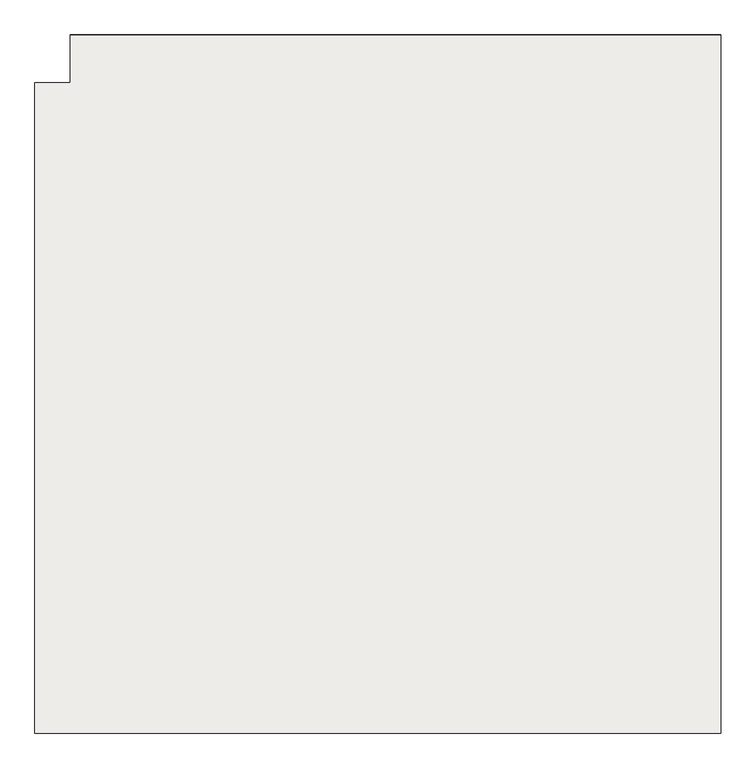
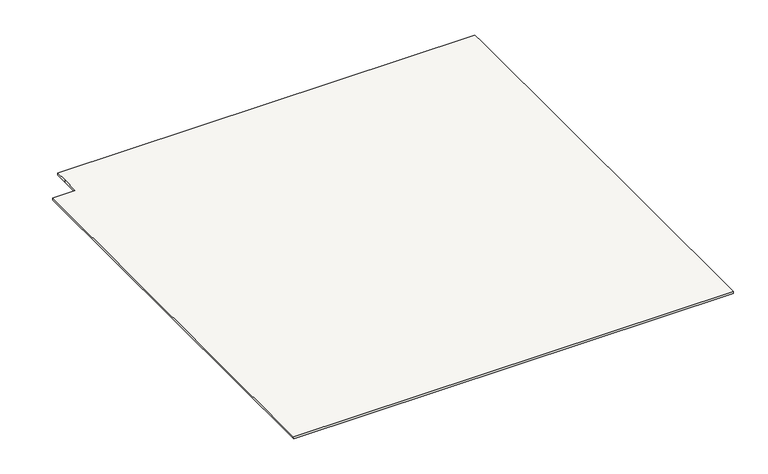
"""IFC4 building model written with IfcOpenShell, lengths in millimetres: slab geometry."""

import ifcopenshell
import ifcopenshell.guid

model = None  # the IFC model being written
_history = None  # IfcOwnerHistory: only IFC2X3 demands one
_inside = {}  # id of a spatial element -> (the spatial element, [elements in it])
_under = {}  # id of a project, library or spatial element -> (it, [spatial elements below it])
_declared = {}  # id of a project -> (the project, [libraries it declares])
_typed = {}  # id of a type object -> (the type object, [elements of that type])
_made_of = {}  # id of a material, layer set ... -> (it, [elements and type objects made of it])


def new_model(schema):
    """Start an empty IFC model of exactly this schema.

    Asked for "IFC4X3", IfcOpenShell would pick the latest addendum, in which some entities
    have other attributes; the version numbers below select the first issue.
    IFC2X3 requires an IfcOwnerHistory on every rooted entity: one is made here for all.
    """
    global model, _history
    if schema == "IFC4X3":
        model = ifcopenshell.file(schema_version=(4, 3, 0, 0))
    else:
        model = ifcopenshell.file(schema=schema)
    _inside.clear()
    _under.clear()
    _declared.clear()
    _typed.clear()
    _made_of.clear()
    _history = None
    if model.schema == "IFC2X3":
        org = make("IfcOrganization", Name="unknown")
        user = make(
            "IfcPersonAndOrganization",
            ThePerson=make("IfcPerson", FamilyName="unknown"),
            TheOrganization=org,
        )
        app = make(
            "IfcApplication",
            ApplicationDeveloper=org,
            Version="unknown",
            ApplicationFullName="unknown",
            ApplicationIdentifier="unknown",
        )
        _history = make(
            "IfcOwnerHistory",
            OwningUser=user,
            OwningApplication=app,
            ChangeAction="ADDED",
            CreationDate=0,
        )
    return model


def make(cls, **values):
    """One entity of the class cls with the attributes given. An attribute that is None is left unset."""
    return model.create_entity(
        cls, **{name: value for name, value in values.items() if value is not None}
    )


def rooted(cls, **values):
    """An entity with a GlobalId (a new one), such as an element, a storey or a relation."""
    return make(cls, GlobalId=ifcopenshell.guid.new(), OwnerHistory=_history, **values)


def si_unit(unit_type, name, prefix=None):
    """IfcSIUnit, for example si_unit("LENGTHUNIT", "METRE", prefix="MILLI")."""
    return make("IfcSIUnit", UnitType=unit_type, Prefix=prefix, Name=name)


def assignment(units):
    """IfcUnitAssignment: the units of a project."""
    return None if units is None else make("IfcUnitAssignment", Units=units)


def point(xyz):
    """IfcCartesianPoint."""
    return None if xyz is None else make("IfcCartesianPoint", Coordinates=xyz)


def direction(xyz):
    """IfcDirection."""
    return None if xyz is None else make("IfcDirection", DirectionRatios=xyz)


def frame(location, z_axis=None, x_axis=None):
    """IfcAxis2Placement3D, a coordinate frame: its origin and axes. An axis left out is left unset."""
    return make(
        "IfcAxis2Placement3D",
        Location=point(location),
        Axis=direction(z_axis),
        RefDirection=direction(x_axis),
    )


def origin():
    """The frame at (0, 0, 0) with its axes left unset."""
    return frame((0.0, 0.0, 0.0))


def place(relative_to, where):
    """IfcLocalPlacement: puts the frame where relative to a parent placement (None: the world)."""
    return make(
        "IfcLocalPlacement", PlacementRelTo=relative_to, RelativePlacement=where
    )


def context(
    kind, dimensions, precision=None, world=None, true_north=None, identifier=None
):
    """IfcGeometricRepresentationContext, for example the 3D "Model" context."""
    return make(
        "IfcGeometricRepresentationContext",
        ContextIdentifier=identifier,
        ContextType=kind,
        CoordinateSpaceDimension=dimensions,
        Precision=precision,
        WorldCoordinateSystem=world,
        TrueNorth=true_north,
    )


def project(units=None, contexts=None):
    """IfcProject with its units and contexts."""
    return rooted(
        "IfcProject",
        Name="project",
        RepresentationContexts=contexts,
        UnitsInContext=assignment(units),
    )


def spatial(cls, under=None, at=None, **own):
    """A site, building, storey or space (cls), placed at a placement, below another one or the project."""
    s = rooted(cls, ObjectPlacement=at, **own)
    if under is not None:
        _under.setdefault(under.id(), (under, []))[1].append(s)
    return s


def faces_of(points, faces, orient=None, outer=None):
    """IfcFace entities. A face is a list of loops; a loop is a list of indices into points, from 0.

    orient and outer hold one flag for each loop. By default every Orientation is true, the
    first loop of a face is its IfcFaceOuterBound and the others are IfcFaceBound.
    """
    made = []
    for i, loops in enumerate(faces):
        bounds = []
        for j, loop in enumerate(loops):
            is_outer = j == 0 if outer is None else outer[i][j]
            bounds.append(
                make(
                    "IfcFaceOuterBound" if is_outer else "IfcFaceBound",
                    Bound=make("IfcPolyLoop", Polygon=[points[k] for k in loop]),
                    Orientation=True if orient is None else orient[i][j],
                )
            )
        made.append(make("IfcFace", Bounds=bounds))
    return made


def faceted_brep(points, faces, orient=None, outer=None, voids=None):
    """IfcFacetedBrep: a solid bounded by flat faces; with voids (closed shells), ...WithVoids."""
    shared = [point(p) for p in points]
    hull = make("IfcClosedShell", CfsFaces=faces_of(shared, faces, orient, outer))
    if voids is None:
        return make("IfcFacetedBrep", Outer=hull)
    return make(
        "IfcFacetedBrepWithVoids",
        Outer=hull,
        Voids=[
            make(cls, CfsFaces=faces_of(shared, fs, o, b)) for cls, fs, o, b in voids
        ],
    )


def shape(context_of_items, identifier, shape_type, items):
    """IfcShapeRepresentation: the items that make up one representation, for example the "Body"."""
    return make(
        "IfcShapeRepresentation",
        ContextOfItems=context_of_items,
        RepresentationIdentifier=identifier,
        RepresentationType=shape_type,
        Items=items,
    )


def source(mapping_origin, context_of_items, identifier, shape_type, items):
    """IfcRepresentationMap: a shape defined once, which mapped items show again and again."""
    return make(
        "IfcRepresentationMap",
        MappingOrigin=mapping_origin,
        MappedRepresentation=shape(context_of_items, identifier, shape_type, items),
    )


def transform(
    local_origin,
    x_axis=None,
    y_axis=None,
    z_axis=None,
    scale=None,
    scale2=None,
    scale3=None,
    uniform=True,
):
    """IfcCartesianTransformationOperator3D, or its non-uniform kind. x_axis, y_axis, z_axis: its Axis1, 2, 3."""
    if uniform:
        return make(
            "IfcCartesianTransformationOperator3D",
            Axis1=direction(x_axis),
            Axis2=direction(y_axis),
            LocalOrigin=point(local_origin),
            Scale=scale,
            Axis3=direction(z_axis),
        )
    return make(
        "IfcCartesianTransformationOperator3DnonUniform",
        Axis1=direction(x_axis),
        Axis2=direction(y_axis),
        LocalOrigin=point(local_origin),
        Scale=scale,
        Axis3=direction(z_axis),
        Scale2=scale2,
        Scale3=scale3,
    )


def mapped(mapping_source, mapping_target):
    """IfcMappedItem: shows the shape of a source again, moved by a transform."""
    return make(
        "IfcMappedItem", MappingSource=mapping_source, MappingTarget=mapping_target
    )


def made_of(thing, what):
    """Note that an element or type object is made of a material, layer set ...; save() writes the relation."""
    if what is not None:
        _made_of.setdefault(what.id(), (what, []))[1].append(thing)
    return thing


def element(
    cls,
    number,
    at=None,
    inside=None,
    cuts=None,
    type_object=None,
    material=None,
    context=None,
    identifier="Body",
    shape_type=None,
    held_by="IfcProductDefinitionShape",
    body=None,
    shapes=None,
    **own,
):
    """One element of the class cls, such as IfcWall. Its Tag is "e" and its number.

    at: its placement. inside: the storey or other place that contains it. cuts: it is an
    opening in that element (IfcRelVoidsElement). A single representation is given by context,
    identifier, shape_type and body (its items); several are given by shapes. held_by: the class
    of the entity that holds the representations. save() writes the other relations.
    """
    e = rooted(cls, Tag="e%d" % number, ObjectPlacement=at, **own)
    if body is not None:
        shapes = [shape(context, identifier, shape_type, body)]
    if shapes is not None:
        e.Representation = make(held_by, Representations=shapes)
    if inside is not None:
        _inside.setdefault(inside.id(), (inside, []))[1].append(e)
    if cuts is not None:
        rooted(
            "IfcRelVoidsElement", RelatingBuildingElement=cuts, RelatedOpeningElement=e
        )
    if type_object is not None:
        _typed.setdefault(type_object.id(), (type_object, []))[1].append(e)
    return made_of(e, material)


def aggregate(whole, parts):
    """IfcRelAggregates: a whole, such as a stair, and the parts it consists of."""
    return rooted("IfcRelAggregates", RelatingObject=whole, RelatedObjects=parts)


def save(model, path):
    """Write the relations noted so far, then the file.

    IfcRelAggregates (storeys below a building ...), IfcRelContainedInSpatialStructure (elements
    in a storey), IfcRelDefinesByType, IfcRelAssociatesMaterial and IfcRelDeclares: one each for
    every whole, place, type object, material and project.
    """
    for whole, parts in _under.values():
        aggregate(whole, parts)
    for where, things in _inside.values():
        rooted(
            "IfcRelContainedInSpatialStructure",
            RelatedElements=things,
            RelatingStructure=where,
        )
    for kind, things in _typed.values():
        rooted("IfcRelDefinesByType", RelatedObjects=things, RelatingType=kind)
    for what, things in _made_of.values():
        rooted("IfcRelAssociatesMaterial", RelatedObjects=things, RelatingMaterial=what)
    for by, libraries in _declared.values():
        rooted("IfcRelDeclares", RelatingContext=by, RelatedDefinitions=libraries)
    model.write(path)


def slab_f74a5215(model_context):
    return source(origin(), model_context, "Body", "Brep", [
        faceted_brep([(16847.5726879, -16667.7074626, 521.7391304), (16847.5726879, -16666.8449626, 515.7391304), (15747.5726879, -16666.8449626, 515.7391304), (15747.5726879, -16667.7074626, 521.7391304), (15687.5726879, -17847.4618478, 521.7391304), (16847.5726879, -17847.4618478, 521.7391304), (16847.5726879, -16698.7691378, 521.7391304), (15747.5726879, -16698.7691378, 521.7391304), (15747.5726879, -16747.4618478, 521.7391304), (15687.5726879, -16747.4618478, 521.7391304), (16847.5726879, -16698.7691378, 515.7391304), (16847.5726879, -17847.4618478, 515.7391304), (15688.4351879, -17847.4618478, 515.7391304), (15688.4351879, -16747.4618478, 515.7391304), (15747.5726879, -16747.4618478, 515.7391304), (15747.5726879, -16698.7691378, 515.7391304)], [[[0, 1, 2, 3]], [[4, 5, 6, 0, 3, 7, 8, 9]], [[10, 11, 12, 13, 14, 15, 2, 1]], [[5, 4, 12, 11]], [[6, 5, 11, 10]], [[0, 6, 10, 1]], [[7, 3, 2, 15]], [[8, 7, 15, 14]], [[9, 8, 14, 13]], [[4, 9, 13, 12]]]),
    ])


if __name__ == "__main__":
    model = new_model("IFC4")
    model_context = context("Model", 3, world=origin())
    ifc_project = project(units=[si_unit("LENGTHUNIT", "METRE", prefix="MILLI")], contexts=[model_context])
    site = spatial("IfcSite", under=ifc_project)
    building = spatial("IfcBuilding", under=site)
    placement = place(None, origin())
    slab_shape = slab_f74a5215(model_context)
    element("IfcSlab", 1, at=placement, inside=building, context=model_context, shape_type="MappedRepresentation", body=[
        mapped(slab_shape, transform((0.0, 0.0, 0.0), x_axis=(1.0, 0.0, 0.0), y_axis=(0.0, 1.0, 0.0), z_axis=(0.0, 0.0, 1.0))),
    ])
    save(model, "model.ifc")

# Revit data of these elements
# Element 1 (IfcSlab)
#   Materials on its faces: "Acero, acabado de pintura, gris oscuro"
# Materials
#   "Acero, acabado de pintura, gris oscuro": class "Metal", colour RGB 89 89 89, transparency 0, Description = "Acero, acabado de pintura, gris oscuro, brillante", Cost = 0
